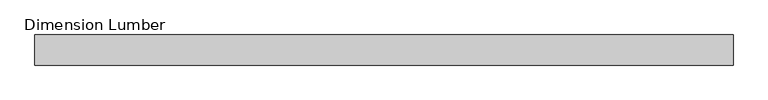
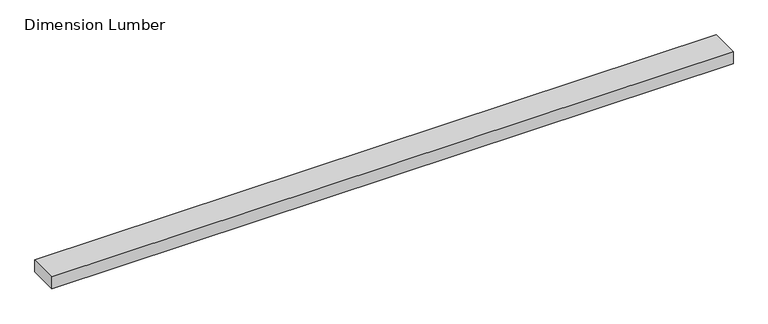
"""IFC4 building model written with IfcOpenShell, lengths in millimetres: beam geometry, Dimension Lumber : Top Supporting Lumbers."""

from ifc_helpers import new_model, si_unit, frame, origin, place, context, project, spatial, polyline, outline, extrude, source, transform, mapped, element, save


def dimension_lumber_59ffca9e(model_context):
    return source(origin(), model_context, "Body", "SweptSolid", [
        extrude(outline(polyline([(1028.7, 44.45), (1028.7, -44.45), (-1028.7, -44.45), (-1028.7, 44.45), (1028.7, 44.45)])), frame((0.0, 0.0, -19.05), z_axis=(0.0, 0.0, 1.0), x_axis=(1.0, 0.0, 0.0)), (0.0, 0.0, 1.0), 38.1),
    ])


if __name__ == "__main__":
    model = new_model("IFC4")
    model_context = context("Model", 3, world=origin())
    ifc_project = project(units=[si_unit("LENGTHUNIT", "METRE", prefix="MILLI")], contexts=[model_context])
    site = spatial("IfcSite", under=ifc_project)
    building = spatial("IfcBuilding", under=site)
    placement = place(None, origin())
    dimension_lumber_shape = dimension_lumber_59ffca9e(model_context)
    element("IfcBeam", 1, ObjectType="Dimension Lumber : Top Supporting Lumbers", at=placement, inside=building, context=model_context, shape_type="MappedRepresentation", body=[
        mapped(dimension_lumber_shape, transform((0.0, 0.0, 0.0), x_axis=(1.0, 0.0, 0.0), y_axis=(0.0, 1.0, 0.0), z_axis=(0.0, 0.0, 1.0))),
    ])
    save(model, "model.ifc")

# Revit data of these elements
# Type "Dimension Lumber : Top Supporting Lumbers"
#   Assembly Code = "B10"
#   A = 0.0364583 SF
#   Length [instance default] = 5' - 0"
#   b = 0' - 3 1/2"
#   d = 0' - 1 1/2"
#   Structural Material [instance default] = Softwood, Lumber
# Element 1 (IfcBeam, "Dimension Lumber : Top Supporting Lumbers")
#   Structural Material = Douglas Fir #2
#   Materials on its faces: "Douglas Fir #2"
# Materials
#   "Softwood, Lumber": class "Wood", colour RGB 223 192 134, transparency 0, Description = "Pinus Echinata", Cost = 0
#   "Douglas Fir #2": class "Wood", colour RGB 223 192 134, transparency 0, Description = "Pinus Echinata", Cost = 0
